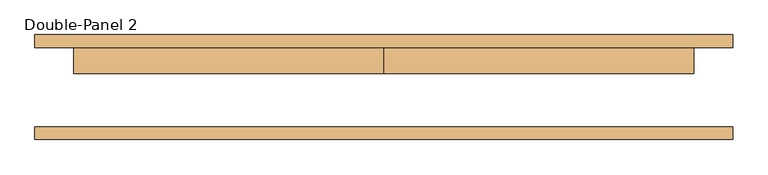
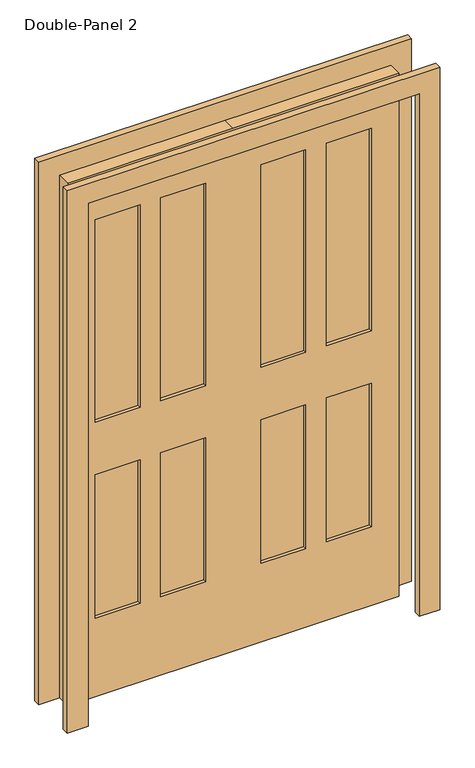
"""IFC4 building model written with IfcOpenShell, lengths in millimetres: door geometry, Double-Panel 2."""

from ifc_helpers import new_model, si_unit, frame, origin, place, context, project, spatial, polyline, outline, extrude, source, transform, mapped, element, save


def double_panel_2_f44b3efe(model_context):
    return source(origin(), model_context, "Body", "SweptSolid", [
        extrude(outline(polyline([(2108.2, -685.8), (0.0, -685.8), (0.0, -609.6), (2032.0, -609.6), (2032.0, 609.6), (0.0, 609.6), (0.0, 685.8), (2108.2, 685.8), (2108.2, -685.8)])), frame((0.0, 77.7875, 0.0), z_axis=(0.0, 1.0, 0.0), x_axis=(0.0, 0.0, 1.0)), (0.0, 0.0, 1.0), 25.4),
        extrude(outline(polyline([(342.9, 65.0875), (508.0, 65.0875), (508.0, 39.6875), (342.9, 39.6875), (342.9, 65.0875)])), frame((0.0, 0.0, 1066.8), z_axis=(0.0, 0.0, 1.0), x_axis=(1.0, 0.0, 0.0)), (0.0, 0.0, 1.0), 787.4),
        extrude(outline(polyline([(101.6, 65.0875), (266.7, 65.0875), (266.7, 39.6875), (101.6, 39.6875), (101.6, 65.0875)])), frame((0.0, 0.0, 1066.8), z_axis=(0.0, 0.0, 1.0), x_axis=(1.0, 0.0, 0.0)), (0.0, 0.0, 1.0), 787.4),
        extrude(outline(polyline([(342.9, 65.0875), (508.0, 65.0875), (508.0, 39.6875), (342.9, 39.6875), (342.9, 65.0875)])), frame((0.0, 0.0, 304.8), z_axis=(0.0, 0.0, 1.0), x_axis=(1.0, 0.0, 0.0)), (0.0, 0.0, 1.0), 558.8),
        extrude(outline(polyline([(101.6, 65.0875), (266.7, 65.0875), (266.7, 39.6875), (101.6, 39.6875), (101.6, 65.0875)])), frame((0.0, 0.0, 304.8), z_axis=(0.0, 0.0, 1.0), x_axis=(1.0, 0.0, 0.0)), (0.0, 0.0, 1.0), 558.8),
        extrude(outline(polyline([(-266.7, 65.0875), (-101.6, 65.0875), (-101.6, 39.6875), (-266.7, 39.6875), (-266.7, 65.0875)])), frame((0.0, 0.0, 1066.8), z_axis=(0.0, 0.0, 1.0), x_axis=(1.0, 0.0, 0.0)), (0.0, 0.0, 1.0), 787.4),
        extrude(outline(polyline([(-508.0, 65.0875), (-342.9, 65.0875), (-342.9, 39.6875), (-508.0, 39.6875), (-508.0, 65.0875)])), frame((0.0, 0.0, 1066.8), z_axis=(0.0, 0.0, 1.0), x_axis=(1.0, 0.0, 0.0)), (0.0, 0.0, 1.0), 787.4),
        extrude(outline(polyline([(-266.7, 65.0875), (-101.6, 65.0875), (-101.6, 39.6875), (-266.7, 39.6875), (-266.7, 65.0875)])), frame((0.0, 0.0, 304.8), z_axis=(0.0, 0.0, 1.0), x_axis=(1.0, 0.0, 0.0)), (0.0, 0.0, 1.0), 558.8),
        extrude(outline(polyline([(-508.0, 65.0875), (-342.9, 65.0875), (-342.9, 39.6875), (-508.0, 39.6875), (-508.0, 65.0875)])), frame((0.0, 0.0, 304.8), z_axis=(0.0, 0.0, 1.0), x_axis=(1.0, 0.0, 0.0)), (0.0, 0.0, 1.0), 558.8),
        extrude(outline(polyline([(2032.0, 0.0), (2032.0, -609.6), (0.0, -609.6), (0.0, 0.0), (0.0, 609.6), (2032.0, 609.6), (2032.0, 0.0)]), holes=[polyline([(1854.2, 342.9), (1854.2, 508.0), (1066.8, 508.0), (1066.8, 342.9), (1854.2, 342.9)]), polyline([(1854.2, 101.6), (1854.2, 266.7), (1066.8, 266.7), (1066.8, 101.6), (1854.2, 101.6)]), polyline([(863.6, 342.9), (863.6, 508.0), (304.8, 508.0), (304.8, 342.9), (863.6, 342.9)]), polyline([(863.6, 101.6), (863.6, 266.7), (304.8, 266.7), (304.8, 101.6), (863.6, 101.6)]), polyline([(1066.8, -266.7), (1854.2, -266.7), (1854.2, -101.6), (1066.8, -101.6), (1066.8, -266.7)]), polyline([(1854.2, -508.0), (1854.2, -342.9), (1066.8, -342.9), (1066.8, -508.0), (1854.2, -508.0)]), polyline([(863.6, -266.7), (863.6, -101.6), (304.8, -101.6), (304.8, -266.7), (863.6, -266.7)]), polyline([(863.6, -508.0), (863.6, -342.9), (304.8, -342.9), (304.8, -508.0), (863.6, -508.0)])]), frame((0.0, 26.9875, 0.0), z_axis=(0.0, 1.0, 0.0), x_axis=(0.0, 0.0, 1.0)), (0.0, 0.0, 1.0), 50.8),
        extrude(outline(polyline([(2032.0, -609.6), (2032.0, 609.6), (0.0, 609.6), (0.0, 685.8), (2108.2, 685.8), (2108.2, -685.8), (0.0, -685.8), (0.0, -609.6), (2032.0, -609.6)])), frame((0.0, -103.1875, 0.0), z_axis=(0.0, 1.0, 0.0), x_axis=(0.0, 0.0, 1.0)), (0.0, 0.0, 1.0), 25.4),
    ])


if __name__ == "__main__":
    model = new_model("IFC4")
    model_context = context("Model", 3, world=origin())
    ifc_project = project(units=[si_unit("LENGTHUNIT", "METRE", prefix="MILLI")], contexts=[model_context])
    site = spatial("IfcSite", under=ifc_project)
    building = spatial("IfcBuilding", under=site)
    placement = place(None, origin())
    double_panel_2_shape = double_panel_2_f44b3efe(model_context)
    element("IfcDoor", 1, ObjectType="Double-Panel 2 : 48\" x 80\"  White", at=placement, inside=building, context=model_context, shape_type="MappedRepresentation", body=[
        mapped(double_panel_2_shape, transform((0.0, 0.0, 0.0), x_axis=(1.0, 0.0, 0.0), y_axis=(0.0, 1.0, 0.0), z_axis=(0.0, 0.0, 1.0))),
    ])
    save(model, "model.ifc")

# Revit data of these elements
# Type "Double-Panel 2 : 48\" x 80\"  White"
#   Type Mark = "84"
#   COBie.Type.CreatedBy = "doug.wood@us.ibm.com"
#   COBie.Type.CreatedOn = "2016-04-14T02:07:24"
#   COBie.Type.Name = "Doors_Double-Panel 2_48\" x 80\"  White_84"
#   COBie.Type.Category = "23-30 10 00 : Doors"
#   COBie.Type.Description = "Double-Panel 2_48\" x 80\"  White"
#   COBie.Type.Manufacturer = ""
#   COBie.Type.ModelNumber = ""
#   Construction Type Id = "MDOOR"
#   Assembly Code = "C1020"
#   Analytic Construction = "Metal"
#   COBie.Type.ReplacementCost = 0
#   Thickness = 0' - 2"
#   Heat Transfer Coefficient (U) = 3.7021 W/(m²·K)
#   Height = 6' - 8"
#   Trim Projection Ext = 0' - 1"
#   Trim Projection Int = 0' - 1"
#   Trim Width = 0' - 3"
#   Width = 4' - 0"
#   COBie.Type = no
#   Door Material = Door - Panel - White
#   Frame Material = Door - Frame - White
#   Visual Light Transmittance = 0
#   Solar Heat Gain Coefficient = 0
#   Function = (empty or 0)
#   Wall Closure = (empty or 0)
# Element 1 (IfcDoor, "Double-Panel 2 : 48\" x 80\"  White")
#   Materials on its faces: "Door - Panel - White", "Door - Frame - White"
# Materials
#   "Door - Panel - White": class "Wood", colour RGB 255 255 255, transparency 0, Cost = 0
#   "Door - Frame - White": class "Miscellaneous", colour RGB 255 255 255, transparency 0, Cost = 0
